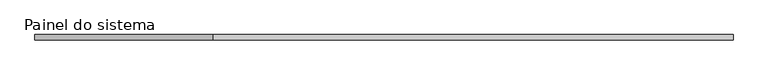
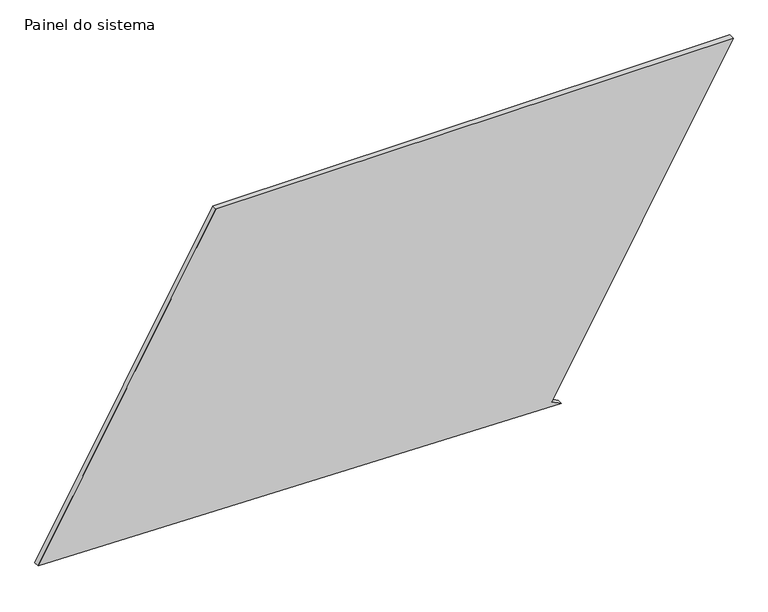
"""IFC4 building model written with IfcOpenShell, lengths in millimetres: plate geometry, Painel do sistema : Envidraçado."""

from ifc_helpers import new_model, si_unit, frame, origin, place, context, project, spatial, polyline, outline, extrude, source, transform, mapped, element, save


def painel_do_sistema_9059aca6(model_context):
    return source(origin(), model_context, "Body", "SweptSolid", [
        extrude(outline(polyline([(0.0, 804.3336826), (24.5641691, 760.7836929), (1495.2562387, 1590.3207146), (1495.2562387, -776.9075122), (53.1502026, -1590.3207146), (0.0, 804.3336826)])), frame((0.0, 24.5, 0.0), z_axis=(0.0, 1.0, 0.0), x_axis=(0.0, 0.0, 1.0)), (0.0, 0.0, 1.0), 25.0),
    ])


if __name__ == "__main__":
    model = new_model("IFC4")
    model_context = context("Model", 3, world=origin())
    ifc_project = project(units=[si_unit("LENGTHUNIT", "METRE", prefix="MILLI")], contexts=[model_context])
    site = spatial("IfcSite", under=ifc_project)
    building = spatial("IfcBuilding", under=site)
    placement = place(None, origin())
    painel_do_sistema_shape = painel_do_sistema_9059aca6(model_context)
    element("IfcPlate", 1, ObjectType="Painel do sistema : Envidraçado", at=placement, inside=building, context=model_context, shape_type="MappedRepresentation", body=[
        mapped(painel_do_sistema_shape, transform((0.0, 0.0, 0.0), x_axis=(1.0, 0.0, 0.0), y_axis=(0.0, 1.0, 0.0), z_axis=(0.0, 0.0, 1.0))),
    ])
    save(model, "model.ifc")

# Revit data of these elements
# Type "Painel do sistema : Envidraçado"
#   Construction Type Id = "GSP4R"
#   Analytic Construction = "Vidraça única Pilkington 1/8 pol"
#   Visual Light Transmittance = 0.9
#   Solar Heat Gain Coefficient = 0.86
#   Heat Transfer Coefficient (U) = 6.7069 W/(m²·K)
# Element 1 (IfcPlate, "Painel do sistema : Envidraçado")
#   Materials on its faces: "Vidro"
# Materials
#   "Vidro": class "Vidro", colour RGB 0 128 192, transparency 0.9, Description = "Vidro de sílica", Cost = 0
